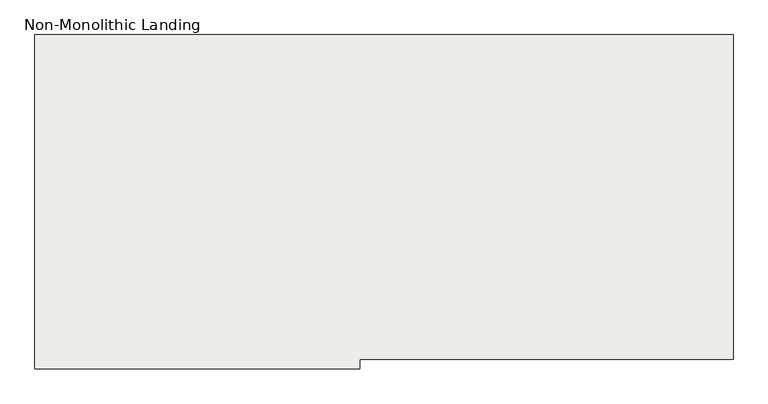
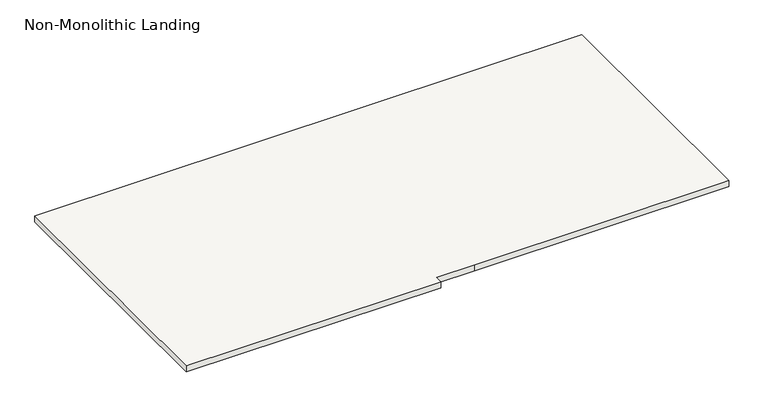
"""IFC4 building model written with IfcOpenShell, lengths in millimetres: slab geometry, Non-Monolithic Landing."""

from ifc_helpers import new_model, si_unit, frame, origin, place, context, project, spatial, polyline, outline, extrude, source, transform, mapped, element, save


def non_monolithic_landing_c55733c2(model_context):
    return source(origin(), model_context, "Body", "SweptSolid", [
        extrude(outline(polyline([(12700.0002443, 23469.9999999), (12700.0002443, 25529.9999999), (17000.0002442, 25529.9999999), (17000.0002442, 23529.9999999), (15000.0002442, 23529.9999999), (14700.0002443, 23529.9999999), (14700.0002443, 23469.9999999), (12700.0002443, 23469.9999999)])), frame((0.0, 0.0, 30450.0), z_axis=(0.0, 0.0, 1.0), x_axis=(1.0, 0.0, 0.0)), (0.0, 0.0, 1.0), 50.0),
    ])


if __name__ == "__main__":
    model = new_model("IFC4")
    model_context = context("Model", 3, world=origin())
    ifc_project = project(units=[si_unit("LENGTHUNIT", "METRE", prefix="MILLI")], contexts=[model_context])
    site = spatial("IfcSite", under=ifc_project)
    building = spatial("IfcBuilding", under=site)
    placement = place(None, origin())
    non_monolithic_landing_shape = non_monolithic_landing_c55733c2(model_context)
    element("IfcSlab", 1, ObjectType="Non-Monolithic Landing", at=placement, inside=building, context=model_context, shape_type="MappedRepresentation", body=[
        mapped(non_monolithic_landing_shape, transform((0.0, 0.0, 0.0), x_axis=(1.0, 0.0, 0.0), y_axis=(0.0, 1.0, 0.0), z_axis=(0.0, 0.0, 1.0))),
    ])
    save(model, "model.ifc")
